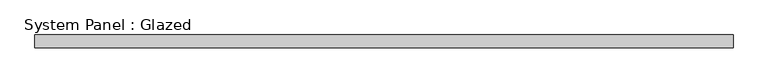
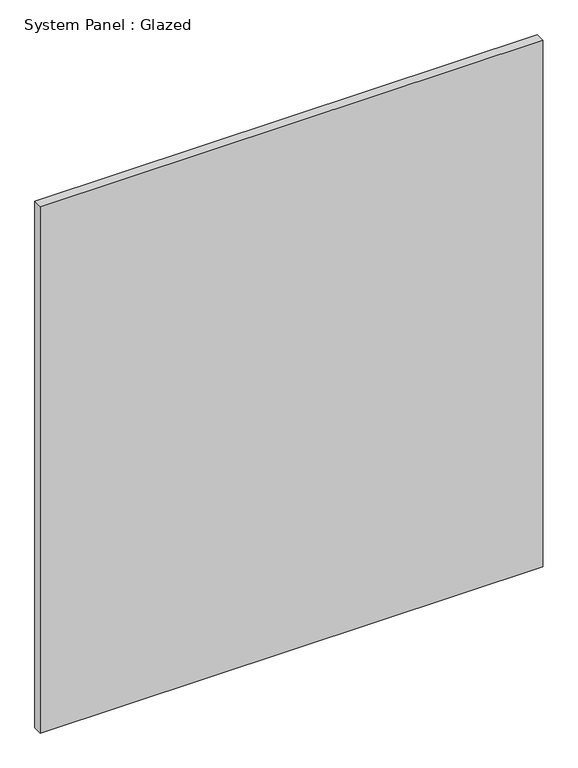
"""IFC4 building model written with IfcOpenShell, lengths in millimetres: plate geometry, System Panel : Glazed."""

from ifc_helpers import new_model, si_unit, origin, origin_with_axes, place, context, project, spatial, polyline, outline, extrude, source, transform, mapped, element, save


def system_panel_glazed_47102c63(model_context):
    return source(origin(), model_context, "Body", "SweptSolid", [
        extrude(outline(polyline([(688.75, 24.5), (-688.75, 24.5), (-688.75, 49.5), (688.75, 49.5), (688.75, 24.5)])), origin_with_axes(), (0.0, 0.0, 1.0), 1526.020449),
    ])


if __name__ == "__main__":
    model = new_model("IFC4")
    model_context = context("Model", 3, world=origin())
    ifc_project = project(units=[si_unit("LENGTHUNIT", "METRE", prefix="MILLI")], contexts=[model_context])
    site = spatial("IfcSite", under=ifc_project)
    building = spatial("IfcBuilding", under=site)
    placement = place(None, origin())
    system_panel_glazed_shape = system_panel_glazed_47102c63(model_context)
    element("IfcPlate", 1, ObjectType="System Panel : Glazed", at=placement, inside=building, context=model_context, shape_type="MappedRepresentation", body=[
        mapped(system_panel_glazed_shape, transform((0.0, 0.0, 0.0), x_axis=(1.0, 0.0, 0.0), y_axis=(0.0, 1.0, 0.0), z_axis=(0.0, 0.0, 1.0))),
    ])
    save(model, "model.ifc")

# Revit data of these elements
# Type "System Panel : Glazed"
#   Keynote = "H11"
#   Construction Type Id = "GSP4R"
#   Analytic Construction = "1/8 in Pilkington single glazing"
#   Visual Light Transmittance = 0.9
#   Solar Heat Gain Coefficient = 0.86
#   Heat Transfer Coefficient (U) = 6.7069 W/(m²·K)
#   Define Thermal Properties by = 1
# Element 1 (IfcPlate, "System Panel : Glazed")
#   Materials on its faces: "Glass"
# Materials
#   "Glass": class "Glass", colour RGB 0 128 192, transparency 0.9, Description = "Soda Lime Glass", Cost = 0
